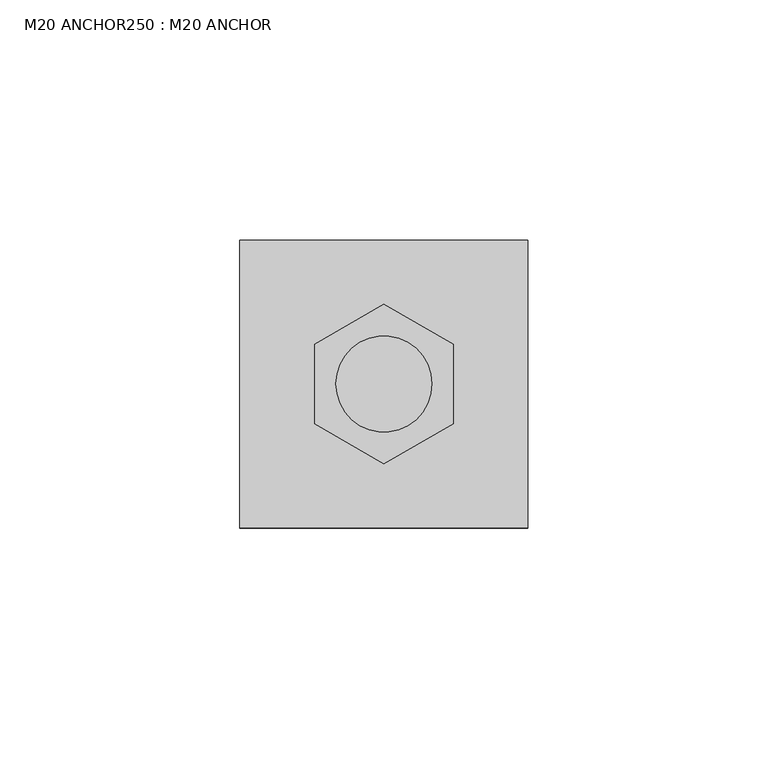
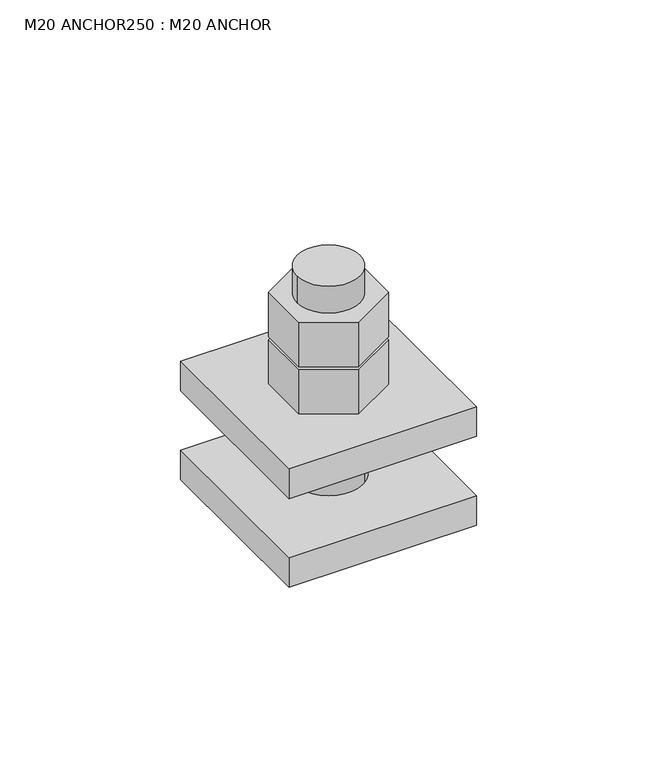
"""IFC4 building model written with IfcOpenShell, lengths in millimetres: fastener geometry, M20 ANCHOR250 : M20 ANCHOR."""

import ifcopenshell
import ifcopenshell.guid

model = None  # the IFC model being written
_history = None  # IfcOwnerHistory: only IFC2X3 demands one
_inside = {}  # id of a spatial element -> (the spatial element, [elements in it])
_under = {}  # id of a project, library or spatial element -> (it, [spatial elements below it])
_declared = {}  # id of a project -> (the project, [libraries it declares])
_typed = {}  # id of a type object -> (the type object, [elements of that type])
_made_of = {}  # id of a material, layer set ... -> (it, [elements and type objects made of it])


def new_model(schema):
    """Start an empty IFC model of exactly this schema.

    Asked for "IFC4X3", IfcOpenShell would pick the latest addendum, in which some entities
    have other attributes; the version numbers below select the first issue.
    IFC2X3 requires an IfcOwnerHistory on every rooted entity: one is made here for all.
    """
    global model, _history
    if schema == "IFC4X3":
        model = ifcopenshell.file(schema_version=(4, 3, 0, 0))
    else:
        model = ifcopenshell.file(schema=schema)
    _inside.clear()
    _under.clear()
    _declared.clear()
    _typed.clear()
    _made_of.clear()
    _history = None
    if model.schema == "IFC2X3":
        org = make("IfcOrganization", Name="unknown")
        user = make(
            "IfcPersonAndOrganization",
            ThePerson=make("IfcPerson", FamilyName="unknown"),
            TheOrganization=org,
        )
        app = make(
            "IfcApplication",
            ApplicationDeveloper=org,
            Version="unknown",
            ApplicationFullName="unknown",
            ApplicationIdentifier="unknown",
        )
        _history = make(
            "IfcOwnerHistory",
            OwningUser=user,
            OwningApplication=app,
            ChangeAction="ADDED",
            CreationDate=0,
        )
    return model


def make(cls, **values):
    """One entity of the class cls with the attributes given. An attribute that is None is left unset."""
    return model.create_entity(
        cls, **{name: value for name, value in values.items() if value is not None}
    )


def rooted(cls, **values):
    """An entity with a GlobalId (a new one), such as an element, a storey or a relation."""
    return make(cls, GlobalId=ifcopenshell.guid.new(), OwnerHistory=_history, **values)


def si_unit(unit_type, name, prefix=None):
    """IfcSIUnit, for example si_unit("LENGTHUNIT", "METRE", prefix="MILLI")."""
    return make("IfcSIUnit", UnitType=unit_type, Prefix=prefix, Name=name)


def assignment(units):
    """IfcUnitAssignment: the units of a project."""
    return None if units is None else make("IfcUnitAssignment", Units=units)


def point(xyz):
    """IfcCartesianPoint."""
    return None if xyz is None else make("IfcCartesianPoint", Coordinates=xyz)


def direction(xyz):
    """IfcDirection."""
    return None if xyz is None else make("IfcDirection", DirectionRatios=xyz)


def frame(location, z_axis=None, x_axis=None):
    """IfcAxis2Placement3D, a coordinate frame: its origin and axes. An axis left out is left unset."""
    return make(
        "IfcAxis2Placement3D",
        Location=point(location),
        Axis=direction(z_axis),
        RefDirection=direction(x_axis),
    )


def frame_2d(location, x_axis=None):
    """IfcAxis2Placement2D, a coordinate frame in the plane: its origin and x axis."""
    return make(
        "IfcAxis2Placement2D", Location=point(location), RefDirection=direction(x_axis)
    )


def origin():
    """The frame at (0, 0, 0) with its axes left unset."""
    return frame((0.0, 0.0, 0.0))


def place(relative_to, where):
    """IfcLocalPlacement: puts the frame where relative to a parent placement (None: the world)."""
    return make(
        "IfcLocalPlacement", PlacementRelTo=relative_to, RelativePlacement=where
    )


def context(
    kind, dimensions, precision=None, world=None, true_north=None, identifier=None
):
    """IfcGeometricRepresentationContext, for example the 3D "Model" context."""
    return make(
        "IfcGeometricRepresentationContext",
        ContextIdentifier=identifier,
        ContextType=kind,
        CoordinateSpaceDimension=dimensions,
        Precision=precision,
        WorldCoordinateSystem=world,
        TrueNorth=true_north,
    )


def project(units=None, contexts=None):
    """IfcProject with its units and contexts."""
    return rooted(
        "IfcProject",
        Name="project",
        RepresentationContexts=contexts,
        UnitsInContext=assignment(units),
    )


def spatial(cls, under=None, at=None, **own):
    """A site, building, storey or space (cls), placed at a placement, below another one or the project."""
    s = rooted(cls, ObjectPlacement=at, **own)
    if under is not None:
        _under.setdefault(under.id(), (under, []))[1].append(s)
    return s


def polyline(points):
    """IfcPolyline through the points."""
    return make("IfcPolyline", Points=[point(p) for p in points])


def circle_curve(where, radius):
    """IfcCircle in the frame where."""
    return make("IfcCircle", Position=where, Radius=radius)


def trimmed(basis, trim1, trim2, sense, master):
    """IfcTrimmedCurve: the piece of a basis curve between two trims."""
    return make(
        "IfcTrimmedCurve",
        BasisCurve=basis,
        Trim1=trim1,
        Trim2=trim2,
        SenseAgreement=sense,
        MasterRepresentation=master,
    )


def segment(curve, same_sense, transition):
    """IfcCompositeCurveSegment."""
    return make(
        "IfcCompositeCurveSegment",
        Transition=transition,
        SameSense=same_sense,
        ParentCurve=curve,
    )


def composite_curve(segments, self_intersect=None):
    """IfcCompositeCurve: segments joined end to end."""
    return make("IfcCompositeCurve", Segments=segments, SelfIntersect=self_intersect)


def outline(outer, holes=None, kind="AREA"):
    """IfcArbitraryClosedProfileDef: a profile drawn as a closed curve; with holes, ...WithVoids."""
    if holes is None:
        return make("IfcArbitraryClosedProfileDef", ProfileType=kind, OuterCurve=outer)
    return make(
        "IfcArbitraryProfileDefWithVoids",
        ProfileType=kind,
        OuterCurve=outer,
        InnerCurves=holes,
    )


def extrude(swept, where, along, depth):
    """IfcExtrudedAreaSolid: the profile swept, set in the frame where, extruded along a direction by depth."""
    return make(
        "IfcExtrudedAreaSolid",
        SweptArea=swept,
        Position=where,
        ExtrudedDirection=direction(along),
        Depth=depth,
    )


def shape(context_of_items, identifier, shape_type, items):
    """IfcShapeRepresentation: the items that make up one representation, for example the "Body"."""
    return make(
        "IfcShapeRepresentation",
        ContextOfItems=context_of_items,
        RepresentationIdentifier=identifier,
        RepresentationType=shape_type,
        Items=items,
    )


def source(mapping_origin, context_of_items, identifier, shape_type, items):
    """IfcRepresentationMap: a shape defined once, which mapped items show again and again."""
    return make(
        "IfcRepresentationMap",
        MappingOrigin=mapping_origin,
        MappedRepresentation=shape(context_of_items, identifier, shape_type, items),
    )


def transform(
    local_origin,
    x_axis=None,
    y_axis=None,
    z_axis=None,
    scale=None,
    scale2=None,
    scale3=None,
    uniform=True,
):
    """IfcCartesianTransformationOperator3D, or its non-uniform kind. x_axis, y_axis, z_axis: its Axis1, 2, 3."""
    if uniform:
        return make(
            "IfcCartesianTransformationOperator3D",
            Axis1=direction(x_axis),
            Axis2=direction(y_axis),
            LocalOrigin=point(local_origin),
            Scale=scale,
            Axis3=direction(z_axis),
        )
    return make(
        "IfcCartesianTransformationOperator3DnonUniform",
        Axis1=direction(x_axis),
        Axis2=direction(y_axis),
        LocalOrigin=point(local_origin),
        Scale=scale,
        Axis3=direction(z_axis),
        Scale2=scale2,
        Scale3=scale3,
    )


def mapped(mapping_source, mapping_target):
    """IfcMappedItem: shows the shape of a source again, moved by a transform."""
    return make(
        "IfcMappedItem", MappingSource=mapping_source, MappingTarget=mapping_target
    )


def made_of(thing, what):
    """Note that an element or type object is made of a material, layer set ...; save() writes the relation."""
    if what is not None:
        _made_of.setdefault(what.id(), (what, []))[1].append(thing)
    return thing


def element(
    cls,
    number,
    at=None,
    inside=None,
    cuts=None,
    type_object=None,
    material=None,
    context=None,
    identifier="Body",
    shape_type=None,
    held_by="IfcProductDefinitionShape",
    body=None,
    shapes=None,
    **own,
):
    """One element of the class cls, such as IfcWall. Its Tag is "e" and its number.

    at: its placement. inside: the storey or other place that contains it. cuts: it is an
    opening in that element (IfcRelVoidsElement). A single representation is given by context,
    identifier, shape_type and body (its items); several are given by shapes. held_by: the class
    of the entity that holds the representations. save() writes the other relations.
    """
    e = rooted(cls, Tag="e%d" % number, ObjectPlacement=at, **own)
    if body is not None:
        shapes = [shape(context, identifier, shape_type, body)]
    if shapes is not None:
        e.Representation = make(held_by, Representations=shapes)
    if inside is not None:
        _inside.setdefault(inside.id(), (inside, []))[1].append(e)
    if cuts is not None:
        rooted(
            "IfcRelVoidsElement", RelatingBuildingElement=cuts, RelatedOpeningElement=e
        )
    if type_object is not None:
        _typed.setdefault(type_object.id(), (type_object, []))[1].append(e)
    return made_of(e, material)


def aggregate(whole, parts):
    """IfcRelAggregates: a whole, such as a stair, and the parts it consists of."""
    return rooted("IfcRelAggregates", RelatingObject=whole, RelatedObjects=parts)


def save(model, path):
    """Write the relations noted so far, then the file.

    IfcRelAggregates (storeys below a building ...), IfcRelContainedInSpatialStructure (elements
    in a storey), IfcRelDefinesByType, IfcRelAssociatesMaterial and IfcRelDeclares: one each for
    every whole, place, type object, material and project.
    """
    for whole, parts in _under.values():
        aggregate(whole, parts)
    for where, things in _inside.values():
        rooted(
            "IfcRelContainedInSpatialStructure",
            RelatedElements=things,
            RelatingStructure=where,
        )
    for kind, things in _typed.values():
        rooted("IfcRelDefinesByType", RelatedObjects=things, RelatingType=kind)
    for what, things in _made_of.values():
        rooted("IfcRelAssociatesMaterial", RelatedObjects=things, RelatingMaterial=what)
    for by, libraries in _declared.values():
        rooted("IfcRelDeclares", RelatingContext=by, RelatedDefinitions=libraries)
    model.write(path)


def m20_anchor250_m20_anchor_728bda02(model_context):
    return source(origin(), model_context, "Body", "SweptSolid", [
        extrude(outline(polyline([(9008.0855968, 22545.0952779), (9022.4937158, 22553.4138093), (9036.9018348, 22545.0952779), (9036.9018348, 22528.4582151), (9022.4937158, 22520.1396837), (9008.0855968, 22528.4582151), (9008.0855968, 22545.0952779)]), holes=[composite_curve([segment(trimmed(circle_curve(frame_2d((9022.4937158, 22536.7767465)), 10.0), [point((9032.4937158, 22536.7767465))], [point((9012.4937158, 22536.7767465))], True, "CARTESIAN"), True, "CONTINUOUS"), segment(trimmed(circle_curve(frame_2d((9022.4937158, 22536.7767465)), 10.0), [point((9012.4937158, 22536.7767465))], [point((9032.4937158, 22536.7767465))], True, "CARTESIAN"), True, "CONTINUOUS")], self_intersect=False)]), frame((0.0, 0.0, 246.0), z_axis=(0.0, 0.0, 1.0), x_axis=(1.0, 0.0, 0.0)), (0.0, 0.0, 1.0), 15.0),
        extrude(outline(polyline([(9008.0855968, 22545.0952779), (9022.4937158, 22553.4138093), (9036.9018348, 22545.0952779), (9036.9018348, 22528.4582151), (9022.4937158, 22520.1396837), (9008.0855968, 22528.4582151), (9008.0855968, 22545.0952779)]), holes=[composite_curve([segment(trimmed(circle_curve(frame_2d((9022.4937158, 22536.7767465)), 10.0), [point((9032.4937158, 22536.7767465))], [point((9012.4937158, 22536.7767465))], True, "CARTESIAN"), True, "CONTINUOUS"), segment(trimmed(circle_curve(frame_2d((9022.4937158, 22536.7767465)), 10.0), [point((9012.4937158, 22536.7767465))], [point((9032.4937158, 22536.7767465))], True, "CARTESIAN"), True, "CONTINUOUS")], self_intersect=False)]), frame((0.0, 0.0, 230.0), z_axis=(0.0, 0.0, 1.0), x_axis=(1.0, 0.0, 0.0)), (0.0, 0.0, 1.0), 15.0),
        extrude(outline(composite_curve([segment(trimmed(circle_curve(frame_2d((9022.4937158, 22536.7767465)), 10.0), [point((9032.4937158, 22536.7767465))], [point((9012.4937158, 22536.7767465))], False, "CARTESIAN"), True, "CONTINUOUS"), segment(trimmed(circle_curve(frame_2d((9022.4937158, 22536.7767465)), 10.0), [point((9012.4937158, 22536.7767465))], [point((9032.4937158, 22536.7767465))], False, "CARTESIAN"), True, "CONTINUOUS")], self_intersect=False)), frame((0.0, 0.0, 190.0), z_axis=(0.0, 0.0, 1.0), x_axis=(1.0, 0.0, 0.0)), (0.0, 0.0, 1.0), 80.0),
        extrude(outline(polyline([(8992.4937158, 22566.7767465), (9052.4937158, 22566.7767465), (9052.4937158, 22506.7767465), (8992.4937158, 22506.7767465), (8992.4937158, 22566.7767465)]), holes=[composite_curve([segment(trimmed(circle_curve(frame_2d((9022.4937158, 22536.7767465)), 11.0), [point((9033.4937158, 22536.7767465))], [point((9011.4937158, 22536.7767465))], True, "CARTESIAN"), True, "CONTINUOUS"), segment(trimmed(circle_curve(frame_2d((9022.4937158, 22536.7767465)), 11.0), [point((9011.4937158, 22536.7767465))], [point((9033.4937158, 22536.7767465))], True, "CARTESIAN"), True, "CONTINUOUS")], self_intersect=False)]), frame((0.0, 0.0, 190.0), z_axis=(0.0, 0.0, 1.0), x_axis=(1.0, 0.0, 0.0)), (0.0, 0.0, 1.0), 10.0),
        extrude(outline(polyline([(8992.4937158, 22566.7767465), (9052.4937158, 22566.7767465), (9052.4937158, 22506.7767465), (8992.4937158, 22506.7767465), (8992.4937158, 22566.7767465)]), holes=[composite_curve([segment(trimmed(circle_curve(frame_2d((9022.4937158, 22536.7767465)), 11.0), [point((9033.4937158, 22536.7767465))], [point((9011.4937158, 22536.7767465))], True, "CARTESIAN"), True, "CONTINUOUS"), segment(trimmed(circle_curve(frame_2d((9022.4937158, 22536.7767465)), 11.0), [point((9011.4937158, 22536.7767465))], [point((9033.4937158, 22536.7767465))], True, "CARTESIAN"), True, "CONTINUOUS")], self_intersect=False)]), frame((0.0, 0.0, 220.0), z_axis=(0.0, 0.0, 1.0), x_axis=(1.0, 0.0, 0.0)), (0.0, 0.0, 1.0), 10.0),
    ])


if __name__ == "__main__":
    model = new_model("IFC4")
    model_context = context("Model", 3, world=origin())
    ifc_project = project(units=[si_unit("LENGTHUNIT", "METRE", prefix="MILLI")], contexts=[model_context])
    site = spatial("IfcSite", under=ifc_project)
    building = spatial("IfcBuilding", under=site)
    placement = place(None, origin())
    m20_anchor250_m20_anchor_shape = m20_anchor250_m20_anchor_728bda02(model_context)
    element("IfcFastener", 1, ObjectType="M20 ANCHOR250 : M20 ANCHOR", at=placement, inside=building, context=model_context, shape_type="MappedRepresentation", body=[
        mapped(m20_anchor250_m20_anchor_shape, transform((0.0, 0.0, 0.0), x_axis=(1.0, 0.0, 0.0), y_axis=(0.0, 1.0, 0.0), z_axis=(0.0, 0.0, 1.0))),
    ])
    save(model, "model.ifc")
